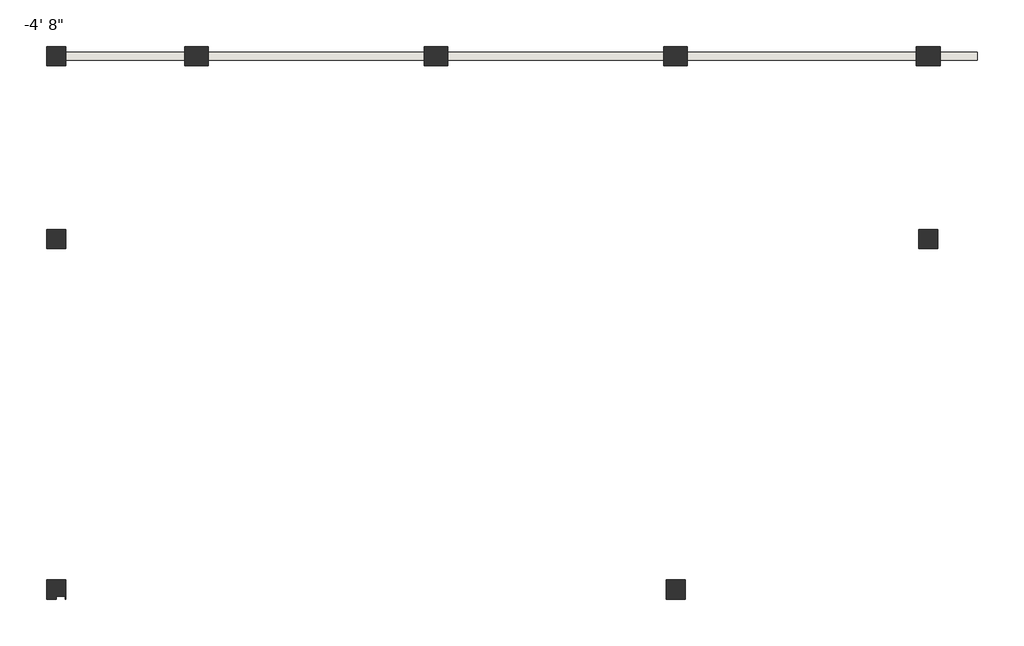
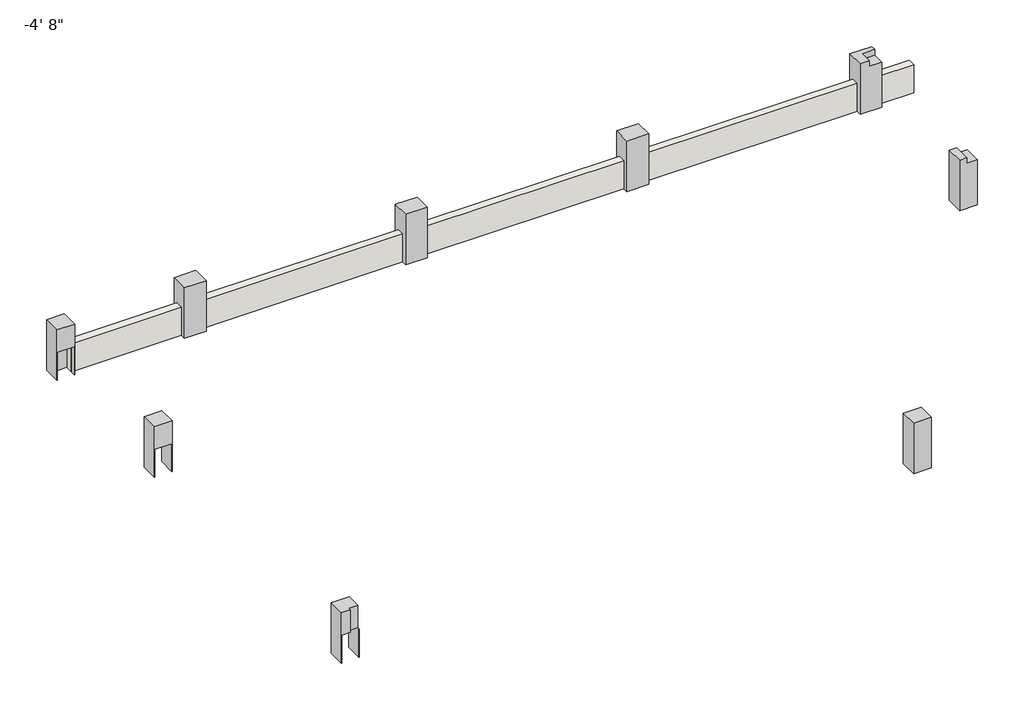
# One storey: 9 columns, 1 wall.
"""IFC4 building model written with IfcOpenShell, lengths in millimetres."""

import ifcopenshell
import ifcopenshell.guid

model = None  # the IFC model being written
_history = None  # IfcOwnerHistory: only IFC2X3 demands one
_inside = {}  # id of a spatial element -> (the spatial element, [elements in it])
_under = {}  # id of a project, library or spatial element -> (it, [spatial elements below it])
_declared = {}  # id of a project -> (the project, [libraries it declares])
_typed = {}  # id of a type object -> (the type object, [elements of that type])
_made_of = {}  # id of a material, layer set ... -> (it, [elements and type objects made of it])


def new_model(schema):
    """Start an empty IFC model of exactly this schema.

    Asked for "IFC4X3", IfcOpenShell would pick the latest addendum, in which some entities
    have other attributes; the version numbers below select the first issue.
    IFC2X3 requires an IfcOwnerHistory on every rooted entity: one is made here for all.
    """
    global model, _history
    if schema == "IFC4X3":
        model = ifcopenshell.file(schema_version=(4, 3, 0, 0))
    else:
        model = ifcopenshell.file(schema=schema)
    _inside.clear()
    _under.clear()
    _declared.clear()
    _typed.clear()
    _made_of.clear()
    _history = None
    if model.schema == "IFC2X3":
        org = make("IfcOrganization", Name="unknown")
        user = make(
            "IfcPersonAndOrganization",
            ThePerson=make("IfcPerson", FamilyName="unknown"),
            TheOrganization=org,
        )
        app = make(
            "IfcApplication",
            ApplicationDeveloper=org,
            Version="unknown",
            ApplicationFullName="unknown",
            ApplicationIdentifier="unknown",
        )
        _history = make(
            "IfcOwnerHistory",
            OwningUser=user,
            OwningApplication=app,
            ChangeAction="ADDED",
            CreationDate=0,
        )
    return model


def make(cls, **values):
    """One entity of the class cls with the attributes given. An attribute that is None is left unset."""
    return model.create_entity(
        cls, **{name: value for name, value in values.items() if value is not None}
    )


def rooted(cls, **values):
    """An entity with a GlobalId (a new one), such as an element, a storey or a relation."""
    return make(cls, GlobalId=ifcopenshell.guid.new(), OwnerHistory=_history, **values)


def si_unit(unit_type, name, prefix=None):
    """IfcSIUnit, for example si_unit("LENGTHUNIT", "METRE", prefix="MILLI")."""
    return make("IfcSIUnit", UnitType=unit_type, Prefix=prefix, Name=name)


def assignment(units):
    """IfcUnitAssignment: the units of a project."""
    return None if units is None else make("IfcUnitAssignment", Units=units)


def point(xyz):
    """IfcCartesianPoint."""
    return None if xyz is None else make("IfcCartesianPoint", Coordinates=xyz)


def direction(xyz):
    """IfcDirection."""
    return None if xyz is None else make("IfcDirection", DirectionRatios=xyz)


def frame(location, z_axis=None, x_axis=None):
    """IfcAxis2Placement3D, a coordinate frame: its origin and axes. An axis left out is left unset."""
    return make(
        "IfcAxis2Placement3D",
        Location=point(location),
        Axis=direction(z_axis),
        RefDirection=direction(x_axis),
    )


def origin():
    """The frame at (0, 0, 0) with its axes left unset."""
    return frame((0.0, 0.0, 0.0))


def place(relative_to, where):
    """IfcLocalPlacement: puts the frame where relative to a parent placement (None: the world)."""
    return make(
        "IfcLocalPlacement", PlacementRelTo=relative_to, RelativePlacement=where
    )


def context(
    kind, dimensions, precision=None, world=None, true_north=None, identifier=None
):
    """IfcGeometricRepresentationContext, for example the 3D "Model" context."""
    return make(
        "IfcGeometricRepresentationContext",
        ContextIdentifier=identifier,
        ContextType=kind,
        CoordinateSpaceDimension=dimensions,
        Precision=precision,
        WorldCoordinateSystem=world,
        TrueNorth=true_north,
    )


def project(units=None, contexts=None):
    """IfcProject with its units and contexts."""
    return rooted(
        "IfcProject",
        Name="project",
        RepresentationContexts=contexts,
        UnitsInContext=assignment(units),
    )


def spatial(cls, under=None, at=None, **own):
    """A site, building, storey or space (cls), placed at a placement, below another one or the project."""
    s = rooted(cls, ObjectPlacement=at, **own)
    if under is not None:
        _under.setdefault(under.id(), (under, []))[1].append(s)
    return s


def polyline(points):
    """IfcPolyline through the points."""
    return make("IfcPolyline", Points=[point(p) for p in points])


def outline(outer, holes=None, kind="AREA"):
    """IfcArbitraryClosedProfileDef: a profile drawn as a closed curve; with holes, ...WithVoids."""
    if holes is None:
        return make("IfcArbitraryClosedProfileDef", ProfileType=kind, OuterCurve=outer)
    return make(
        "IfcArbitraryProfileDefWithVoids",
        ProfileType=kind,
        OuterCurve=outer,
        InnerCurves=holes,
    )


def extrude(swept, where, along, depth):
    """IfcExtrudedAreaSolid: the profile swept, set in the frame where, extruded along a direction by depth."""
    return make(
        "IfcExtrudedAreaSolid",
        SweptArea=swept,
        Position=where,
        ExtrudedDirection=direction(along),
        Depth=depth,
    )


def faces_of(points, faces, orient=None, outer=None):
    """IfcFace entities. A face is a list of loops; a loop is a list of indices into points, from 0.

    orient and outer hold one flag for each loop. By default every Orientation is true, the
    first loop of a face is its IfcFaceOuterBound and the others are IfcFaceBound.
    """
    made = []
    for i, loops in enumerate(faces):
        bounds = []
        for j, loop in enumerate(loops):
            is_outer = j == 0 if outer is None else outer[i][j]
            bounds.append(
                make(
                    "IfcFaceOuterBound" if is_outer else "IfcFaceBound",
                    Bound=make("IfcPolyLoop", Polygon=[points[k] for k in loop]),
                    Orientation=True if orient is None else orient[i][j],
                )
            )
        made.append(make("IfcFace", Bounds=bounds))
    return made


def faceted_brep(points, faces, orient=None, outer=None, voids=None):
    """IfcFacetedBrep: a solid bounded by flat faces; with voids (closed shells), ...WithVoids."""
    shared = [point(p) for p in points]
    hull = make("IfcClosedShell", CfsFaces=faces_of(shared, faces, orient, outer))
    if voids is None:
        return make("IfcFacetedBrep", Outer=hull)
    return make(
        "IfcFacetedBrepWithVoids",
        Outer=hull,
        Voids=[
            make(cls, CfsFaces=faces_of(shared, fs, o, b)) for cls, fs, o, b in voids
        ],
    )


def shape(context_of_items, identifier, shape_type, items):
    """IfcShapeRepresentation: the items that make up one representation, for example the "Body"."""
    return make(
        "IfcShapeRepresentation",
        ContextOfItems=context_of_items,
        RepresentationIdentifier=identifier,
        RepresentationType=shape_type,
        Items=items,
    )


def source(mapping_origin, context_of_items, identifier, shape_type, items):
    """IfcRepresentationMap: a shape defined once, which mapped items show again and again."""
    return make(
        "IfcRepresentationMap",
        MappingOrigin=mapping_origin,
        MappedRepresentation=shape(context_of_items, identifier, shape_type, items),
    )


def transform(
    local_origin,
    x_axis=None,
    y_axis=None,
    z_axis=None,
    scale=None,
    scale2=None,
    scale3=None,
    uniform=True,
):
    """IfcCartesianTransformationOperator3D, or its non-uniform kind. x_axis, y_axis, z_axis: its Axis1, 2, 3."""
    if uniform:
        return make(
            "IfcCartesianTransformationOperator3D",
            Axis1=direction(x_axis),
            Axis2=direction(y_axis),
            LocalOrigin=point(local_origin),
            Scale=scale,
            Axis3=direction(z_axis),
        )
    return make(
        "IfcCartesianTransformationOperator3DnonUniform",
        Axis1=direction(x_axis),
        Axis2=direction(y_axis),
        LocalOrigin=point(local_origin),
        Scale=scale,
        Axis3=direction(z_axis),
        Scale2=scale2,
        Scale3=scale3,
    )


def mapped(mapping_source, mapping_target):
    """IfcMappedItem: shows the shape of a source again, moved by a transform."""
    return make(
        "IfcMappedItem", MappingSource=mapping_source, MappingTarget=mapping_target
    )


def made_of(thing, what):
    """Note that an element or type object is made of a material, layer set ...; save() writes the relation."""
    if what is not None:
        _made_of.setdefault(what.id(), (what, []))[1].append(thing)
    return thing


def element(
    cls,
    number,
    at=None,
    inside=None,
    cuts=None,
    type_object=None,
    material=None,
    context=None,
    identifier="Body",
    shape_type=None,
    held_by="IfcProductDefinitionShape",
    body=None,
    shapes=None,
    **own,
):
    """One element of the class cls, such as IfcWall. Its Tag is "e" and its number.

    at: its placement. inside: the storey or other place that contains it. cuts: it is an
    opening in that element (IfcRelVoidsElement). A single representation is given by context,
    identifier, shape_type and body (its items); several are given by shapes. held_by: the class
    of the entity that holds the representations. save() writes the other relations.
    """
    e = rooted(cls, Tag="e%d" % number, ObjectPlacement=at, **own)
    if body is not None:
        shapes = [shape(context, identifier, shape_type, body)]
    if shapes is not None:
        e.Representation = make(held_by, Representations=shapes)
    if inside is not None:
        _inside.setdefault(inside.id(), (inside, []))[1].append(e)
    if cuts is not None:
        rooted(
            "IfcRelVoidsElement", RelatingBuildingElement=cuts, RelatedOpeningElement=e
        )
    if type_object is not None:
        _typed.setdefault(type_object.id(), (type_object, []))[1].append(e)
    return made_of(e, material)


def aggregate(whole, parts):
    """IfcRelAggregates: a whole, such as a stair, and the parts it consists of."""
    return rooted("IfcRelAggregates", RelatingObject=whole, RelatedObjects=parts)


def save(model, path):
    """Write the relations noted so far, then the file.

    IfcRelAggregates (storeys below a building ...), IfcRelContainedInSpatialStructure (elements
    in a storey), IfcRelDefinesByType, IfcRelAssociatesMaterial and IfcRelDeclares: one each for
    every whole, place, type object, material and project.
    """
    for whole, parts in _under.values():
        aggregate(whole, parts)
    for where, things in _inside.values():
        rooted(
            "IfcRelContainedInSpatialStructure",
            RelatedElements=things,
            RelatingStructure=where,
        )
    for kind, things in _typed.values():
        rooted("IfcRelDefinesByType", RelatedObjects=things, RelatingType=kind)
    for what, things in _made_of.values():
        rooted("IfcRelAssociatesMaterial", RelatedObjects=things, RelatingMaterial=what)
    for by, libraries in _declared.values():
        rooted("IfcRelDeclares", RelatingContext=by, RelatedDefinitions=libraries)
    model.write(path)


def concrete_rectangular_column_p1_c4786f08(model_context):
    return source(origin(), model_context, "Body", "SweptSolid", [
        extrude(outline(polyline([(228.6, 228.6), (228.6, -228.6), (-228.6, -228.6), (-228.6, 228.6), (228.6, 228.6)])), frame((0.0, 0.0, -1371.6), z_axis=(0.0, 0.0, 1.0), x_axis=(1.0, 0.0, 0.0)), (0.0, 0.0, 1.0), 1371.6),
    ])


model = new_model("IFC4")

# Units and contexts
model_context = context("Model", 3, world=origin())
ifc_project = project(units=[si_unit("LENGTHUNIT", "METRE", prefix="MILLI")], contexts=[model_context])

# Site, building, storey
site = spatial("IfcSite", under=ifc_project)
building = spatial("IfcBuilding", under=site)
storey = spatial("IfcBuildingStorey", under=building, Name="-4' 8\"", Elevation=-1371.6)

# Columns
placement = place(None, origin())
element("IfcColumn", 1, ObjectType="Concrete-Rectangular-Column : P1", at=placement, inside=storey, context=model_context, shape_type="Brep", body=[
    faceted_brep([(-30777.7674689, 8890.1676661, -1371.6), (-30777.7674689, 9347.3676661, -1371.6), (-30320.5674689, 9347.3676661, -1371.6), (-30320.5674689, 9215.6051661, -1371.6), (-30330.0924689, 9215.6051661, -1371.6), (-30768.2424689, 9215.6051661, -1371.6), (-30768.2424689, 8890.1676661, -1371.6), (-30320.5674689, 9347.3676661, 0.0), (-30320.5674689, 8890.1676661, 0.0), (-30320.5674689, 8890.1676661, -1371.6), (-30320.5674689, 9021.9301661, -1371.6), (-30320.5674689, 9021.9301661, -609.6), (-30320.5674689, 9215.6051661, -609.6), (-30777.7674689, 8890.1676661, 0.0), (-30768.2424689, 8890.1676661, -609.6), (-30330.0924689, 8890.1676661, -609.6), (-30330.0924689, 8890.1676661, -1371.6), (-30777.7674689, 9347.3676661, 0.0), (-30330.0924689, 9021.9301661, -609.6), (-30330.0924689, 9021.9301661, -1371.6), (-30768.2424689, 9215.6051661, -609.6), (-30330.0924689, 9215.6051661, -609.6)], [[[0, 1, 2, 3, 4, 5, 6]], [[7, 8, 9, 10, 11, 12, 3, 2]], [[9, 8, 13, 0, 6, 14, 15, 16]], [[1, 0, 13, 17]], [[2, 1, 17, 7]], [[8, 7, 17, 13]], [[16, 15, 18, 19]], [[5, 20, 14, 6]], [[12, 11, 18, 15, 14, 20, 21]], [[12, 21, 20, 5, 4, 3]], [[18, 11, 10, 19]], [[9, 16, 19, 10]]]),
])
element("IfcColumn", 2, ObjectType="Concrete-Rectangular-Column : P1", at=placement, inside=storey, context=model_context, shape_type="SweptSolid", body=[
    extrude(outline(polyline([(-1371.6, -10076.7674689), (-1371.6, -9619.5674689), (-152.4, -9619.5674689), (-152.4, -9889.4424689), (0.0, -9889.4424689), (0.0, -10076.7674689), (-1371.6, -10076.7674689)])), frame((0.0, 4546.7676661, 0.0), z_axis=(0.0, 1.0, 0.0), x_axis=(0.0, 0.0, 1.0)), (0.0, 0.0, 1.0), 457.2),
])
element("IfcColumn", 3, ObjectType="Concrete-Rectangular-Column : P1", at=placement, inside=storey, context=model_context, shape_type="SweptSolid", body=[
    extrude(outline(polyline([(-1371.6, -30320.5674689), (0.0, -30320.5674689), (0.0, -30777.7674689), (-1371.6, -30777.7674689), (-1371.6, -30768.2424689), (-609.6, -30768.2424689), (-609.6, -30330.0924689), (-1371.6, -30330.0924689), (-1371.6, -30320.5674689)])), frame((0.0, 4546.7676661, 0.0), z_axis=(0.0, 1.0, 0.0), x_axis=(0.0, 0.0, 1.0)), (0.0, 0.0, 1.0), 457.2),
])
element("IfcColumn", 4, ObjectType="Concrete-Rectangular-Column : P1", at=placement, inside=storey, context=model_context, shape_type="Brep", body=[
    faceted_brep([(-30777.7674689, -3784.4323339, -1371.6), (-30777.7674689, -3327.2323339, -1371.6), (-30768.2424689, -3327.2323339, -1371.6), (-30768.2424689, -3784.4323339, -1371.6), (-30320.5674689, -3784.4323339, -1371.6), (-30320.5674689, -3327.2323339, -1371.6), (-30320.5674689, -3327.2323339, 0.0), (-30320.5674689, -3708.2323339, 0.0), (-30320.5674689, -3708.2323339, -609.6), (-30320.5674689, -3784.4323339, -609.6), (-30777.7674689, -3784.4323339, 0.0), (-30768.2424689, -3784.4323339, -609.6), (-30549.1674689, -3784.4323339, -609.6), (-30549.1674689, -3784.4323339, 0.0), (-30777.7674689, -3327.2323339, 0.0), (-30330.0924689, -3327.2323339, -1371.6), (-30330.0924689, -3327.2323339, -609.6), (-30768.2424689, -3327.2323339, -609.6), (-30549.1674689, -3708.2323339, 0.0), (-30330.0924689, -3784.4323339, -1371.6), (-30330.0924689, -3784.4323339, -609.6), (-30330.0924689, -3708.2323339, -609.6), (-30549.1674689, -3708.2323339, -609.6)], [[[0, 1, 2, 3]], [[4, 5, 6, 7, 8, 9]], [[10, 0, 3, 11, 12, 13]], [[1, 0, 10, 14]], [[6, 5, 15, 16, 17, 2, 1, 14]], [[14, 10, 13, 18, 7, 6]], [[15, 19, 20, 21, 16]], [[17, 11, 3, 2]], [[11, 17, 16, 21, 22, 12]], [[5, 4, 19, 15]], [[21, 8, 7, 18, 22]], [[8, 21, 20, 9]], [[22, 18, 13, 12]], [[19, 4, 9, 20]]]),
])
concrete_rectangular_column_p1_shape = concrete_rectangular_column_p1_c4786f08(model_context)
element("IfcColumn", 5, ObjectType="Concrete-Rectangular-Column : P1", at=placement, inside=storey, context=model_context, shape_type="MappedRepresentation", body=[
    mapped(concrete_rectangular_column_p1_shape, transform((-15842.5674689, -3555.8323339, 0.0), x_axis=(1.0, 0.0, 0.0), y_axis=(0.0, 1.0, 0.0), z_axis=(0.0, 0.0, 1.0))),
])
element("IfcColumn", 6, ObjectType="Concrete-Rectangular-Column : P2", at=placement, inside=storey, context=model_context, shape_type="SweptSolid", body=[
    extrude(outline(polyline([(8890.1676661, -1371.6), (8890.1676661, 0.0), (9347.3676661, 0.0), (9347.3676661, -1371.6), (9215.6051661, -1371.6), (9215.6051661, -609.6), (9021.9301661, -609.6), (9021.9301661, -1371.6), (8890.1676661, -1371.6)])), frame((-27501.1674689, 0.0, 0.0), z_axis=(1.0, 0.0, 0.0), x_axis=(0.0, 1.0, 0.0)), (0.0, 0.0, 1.0), 558.8),
])
element("IfcColumn", 7, ObjectType="Concrete-Rectangular-Column : P2", at=placement, inside=storey, context=model_context, shape_type="SweptSolid", body=[
    extrude(outline(polyline([(8890.1676661, -1371.6), (8890.1676661, 0.0), (9347.3676661, 0.0), (9347.3676661, -1371.6), (9215.6051661, -1371.6), (9215.6051661, -609.6), (9021.9301661, -609.6), (9021.9301661, -1371.6), (8890.1676661, -1371.6)])), frame((-21811.5674689, 0.0, 0.0), z_axis=(1.0, 0.0, 0.0), x_axis=(0.0, 1.0, 0.0)), (0.0, 0.0, 1.0), 558.8),
])
element("IfcColumn", 8, ObjectType="Concrete-Rectangular-Column : P2", at=placement, inside=storey, context=model_context, shape_type="SweptSolid", body=[
    extrude(outline(polyline([(8890.1676661, -1371.6), (8890.1676661, 0.0), (9347.3676661, 0.0), (9347.3676661, -1371.6), (9215.6051661, -1371.6), (9215.6051661, -609.6), (9021.9301661, -609.6), (9021.9301661, -1371.6), (8890.1676661, -1371.6)])), frame((-16121.9674689, 0.0, 0.0), z_axis=(1.0, 0.0, 0.0), x_axis=(0.0, 1.0, 0.0)), (0.0, 0.0, 1.0), 558.8),
])
element("IfcColumn", 9, ObjectType="Concrete-Rectangular-Column : P2", at=placement, inside=storey, context=model_context, shape_type="Brep", body=[
    faceted_brep([(-10127.5674689, 9347.3676661, -1371.6), (-9568.7674689, 9347.3676661, -1371.6), (-9568.7674689, 9215.6051661, -1371.6), (-10127.5674689, 9215.6051661, -1371.6), (-9568.7674689, 9347.3676661, 0.0), (-9568.7674689, 9215.6051661, 0.0), (-9568.7674689, 9215.6051661, -152.4), (-9568.7674689, 8890.1676661, -152.4), (-9568.7674689, 8890.1676661, -1371.6), (-9568.7674689, 9021.9301661, -1371.6), (-9568.7674689, 9021.9301661, -609.6), (-9568.7674689, 9215.6051661, -609.6), (-10127.5674689, 8890.1676661, -1371.6), (-9889.4424689, 8890.1676661, -152.4), (-9889.4424689, 8890.1676661, 0.0), (-10127.5674689, 8890.1676661, 0.0), (-10127.5674689, 9347.3676661, 0.0), (-10127.5674689, 9215.6051661, -609.6), (-10127.5674689, 9021.9301661, -609.6), (-10127.5674689, 9021.9301661, -1371.6), (-9889.4424689, 9215.6051661, 0.0), (-9889.4424689, 9215.6051661, -152.4)], [[[0, 1, 2, 3]], [[1, 4, 5, 6, 7, 8, 9, 10, 11, 2]], [[12, 8, 7, 13, 14, 15]], [[12, 15, 16, 0, 3, 17, 18, 19]], [[1, 0, 16, 4]], [[16, 15, 14, 20, 5, 4]], [[6, 21, 13, 7]], [[21, 20, 14, 13]], [[20, 21, 6, 5]], [[18, 10, 9, 19]], [[11, 17, 3, 2]], [[10, 18, 17, 11]], [[8, 12, 19, 9]]]),
])

# Wall
element("IfcWall", 10, ObjectType="Generic - 8\" Masonry", at=placement, inside=storey, context=model_context, shape_type="Brep", body=[
    faceted_brep([(-30330.0924689, 9021.9301661, -1371.6), (-30320.5674689, 9021.9301661, -1371.6), (-27501.1674689, 9021.9301661, -1371.6), (-26942.3674689, 9021.9301661, -1371.6), (-21811.5674689, 9021.9301661, -1371.6), (-21252.7674689, 9021.9301661, -1371.6), (-16121.9674689, 9021.9301661, -1371.6), (-15563.1674689, 9021.9301661, -1371.6), (-10127.5674689, 9021.9301661, -1371.6), (-9568.7674689, 9021.9301661, -1371.6), (-8679.7674689, 9021.9301661, -1371.6), (-8679.7674689, 9021.9301661, -1016.0), (-8679.7674689, 9021.9301661, -647.7), (-8679.7674689, 9021.9301661, -609.6), (-9568.7674689, 9021.9301661, -609.6), (-10127.5674689, 9021.9301661, -609.6), (-15563.1674689, 9021.9301661, -609.6), (-16121.9674689, 9021.9301661, -609.6), (-21252.7674689, 9021.9301661, -609.6), (-21811.5674689, 9021.9301661, -609.6), (-26942.3674689, 9021.9301661, -609.6), (-27501.1674689, 9021.9301661, -609.6), (-30320.5674689, 9021.9301661, -609.6), (-30330.0924689, 9021.9301661, -609.6), (-30330.0924689, 9215.6051661, -1371.6), (-30330.0924689, 9215.6051661, -609.6), (-30320.5674689, 9215.6051661, -609.6), (-27501.1674689, 9215.6051661, -609.6), (-26942.3674689, 9215.6051661, -609.6), (-21811.5674689, 9215.6051661, -609.6), (-21252.7674689, 9215.6051661, -609.6), (-16121.9674689, 9215.6051661, -609.6), (-15563.1674689, 9215.6051661, -609.6), (-10127.5674689, 9215.6051661, -609.6), (-9568.7674689, 9215.6051661, -609.6), (-8679.7674689, 9215.6051661, -609.6), (-8679.7674689, 9215.6051661, -647.7), (-8679.7674689, 9215.6051661, -1016.0), (-8679.7674689, 9215.6051661, -1371.6), (-9568.7674689, 9215.6051661, -1371.6), (-10127.5674689, 9215.6051661, -1371.6), (-15563.1674689, 9215.6051661, -1371.6), (-16121.9674689, 9215.6051661, -1371.6), (-21252.7674689, 9215.6051661, -1371.6), (-21811.5674689, 9215.6051661, -1371.6), (-26942.3674689, 9215.6051661, -1371.6), (-27501.1674689, 9215.6051661, -1371.6), (-30320.5674689, 9215.6051661, -1371.6)], [[[0, 1, 2, 3, 4, 5, 6, 7, 8, 9, 10, 11, 12, 13, 14, 15, 16, 17, 18, 19, 20, 21, 22, 23]], [[24, 25, 26, 27, 28, 29, 30, 31, 32, 33, 34, 35, 36, 37, 38, 39, 40, 41, 42, 43, 44, 45, 46, 47]], [[10, 9, 8, 7, 6, 5, 4, 3, 2, 1, 0, 24, 47, 46, 45, 44, 43, 42, 41, 40, 39, 38]], [[13, 12, 11, 10, 38, 37, 36, 35]], [[23, 22, 21, 20, 19, 18, 17, 16, 15, 14, 13, 35, 34, 33, 32, 31, 30, 29, 28, 27, 26, 25]], [[0, 23, 25, 24]]]),
])

save(model, "model.ifc")

# Revit data of these elements
# Type "Concrete-Rectangular-Column : P1"
#   Assembly Code = "B10"
#   b = 1' - 6"
#   h = 1' - 6"
#   Structural Material [instance default] = Concrete, Cast-in-Place gray
# Type "Concrete-Rectangular-Column : P2"
#   Assembly Code = "B10"
#   b = 1' - 10"
#   h = 1' - 6"
#   Structural Material [instance default] = Concrete, Cast-in-Place gray
# Type "Generic - 8\" Masonry"
#   Assembly Code = "B2010"
#   Layers, outside or top first: 0' - 7 5/8" "Concrete Masonry Units" (function 1)
# Elements 1, 2, 3, 4, 5 (IfcColumn, "Concrete-Rectangular-Column : P1")
#   Comments = ""
#   Structural Material = Concrete, Cast-in-Place gray
#   Phase Created = New Construction
#   Materials on its faces: "Concrete, Cast-in-Place gray"
# Elements 6, 7, 8, 9 (IfcColumn, "Concrete-Rectangular-Column : P2")
#   Comments = ""
#   Structural Material = Concrete, Cast-in-Place gray
#   Phase Created = New Construction
#   Materials on its faces: "Concrete, Cast-in-Place gray"
# Element 10 (IfcWall, "Generic - 8\" Masonry")
#   Comments = ""
#   Top Offset = -2' - 0"
#   Base Offset = 0' - 0"
#   wall height = 2' - 6"
#   Phase Created = New Construction
#   Base Constraint = -4' 8"
#   Top Constraint = Level 1
#   Materials on its faces: "Concrete Masonry Units"
# Materials
#   "Concrete, Cast-in-Place gray": class "Concrete", colour RGB 192 192 192, transparency 0, Description = "Cast-in-place concrete", Cost = 0
#   "Concrete Masonry Units": class "Masonry", colour RGB 227 227 227, transparency 0, Description = "Concrete masonry units", Cost = 0
